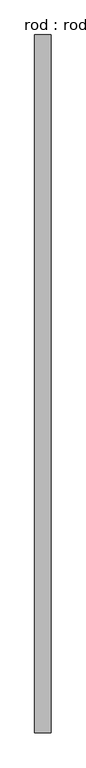
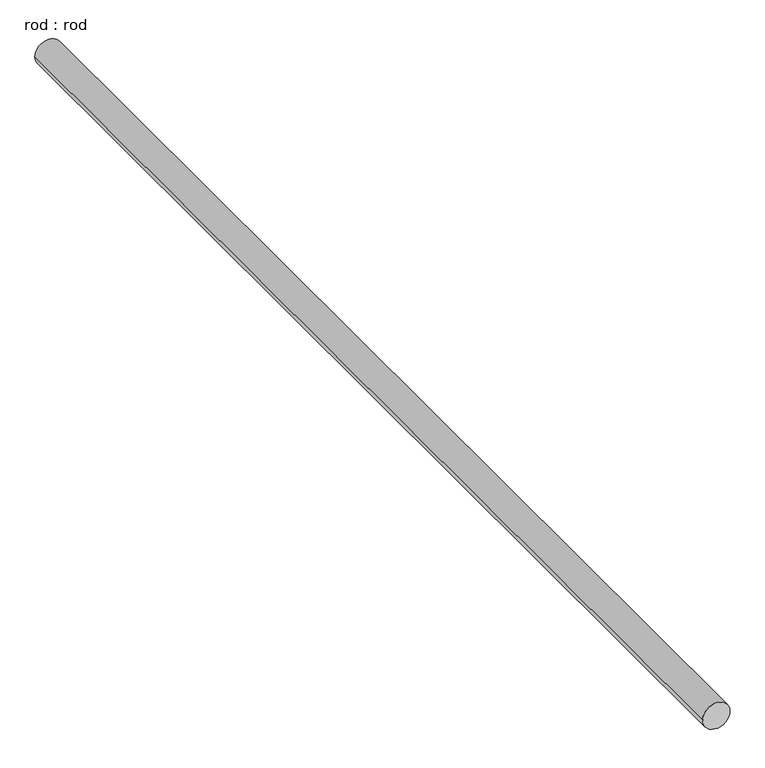
"""IFC4 building model written with IfcOpenShell, lengths in millimetres: proxy geometry, rod : rod."""

from ifc_helpers import new_model, si_unit, point, frame, frame_2d, origin, place, context, project, spatial, circle_curve, trimmed, segment, composite_curve, outline, extrude, source, transform, mapped, element, save


def rod_rod_65aaeb38(model_context):
    return source(origin(), model_context, "Body", "SweptSolid", [
        extrude(outline(composite_curve([segment(trimmed(circle_curve(frame_2d((0.0108462, 0.0)), 200.0), [point((0.0108462, 200.0))], [point((0.0108462, -200.0))], False, "CARTESIAN"), True, "CONTINUOUS"), segment(trimmed(circle_curve(frame_2d((0.0108462, 0.0)), 200.0), [point((0.0108462, -200.0))], [point((0.0108462, 200.0))], False, "CARTESIAN"), True, "CONTINUOUS")], self_intersect=False)), frame((0.0, -4398.3428132, 0.0), z_axis=(0.0, 1.0, 0.0), x_axis=(0.0, 0.0, 1.0)), (0.0, 0.0, 1.0), 16982.1428571),
    ])


if __name__ == "__main__":
    model = new_model("IFC4")
    model_context = context("Model", 3, world=origin())
    ifc_project = project(units=[si_unit("LENGTHUNIT", "METRE", prefix="MILLI")], contexts=[model_context])
    site = spatial("IfcSite", under=ifc_project)
    building = spatial("IfcBuilding", under=site)
    placement = place(None, origin())
    rod_rod_shape = rod_rod_65aaeb38(model_context)
    element("IfcBuildingElementProxy", 1, Name="rod : rod", ObjectType="rod : rod", at=placement, inside=building, context=model_context, shape_type="MappedRepresentation", body=[
        mapped(rod_rod_shape, transform((0.0, 0.0, 0.0), x_axis=(1.0, 0.0, 0.0), y_axis=(0.0, 1.0, 0.0), z_axis=(0.0, 0.0, 1.0))),
    ])
    save(model, "model.ifc")

# Revit data of these elements
# Type "rod : rod"
#   Default Elevation = 0
